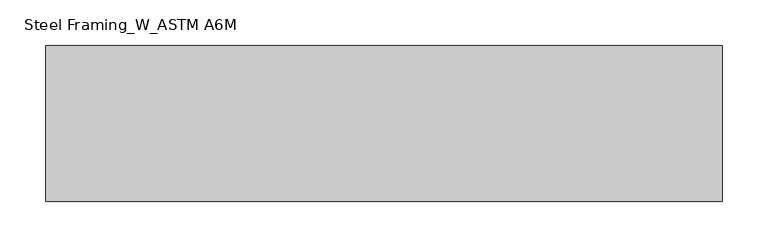
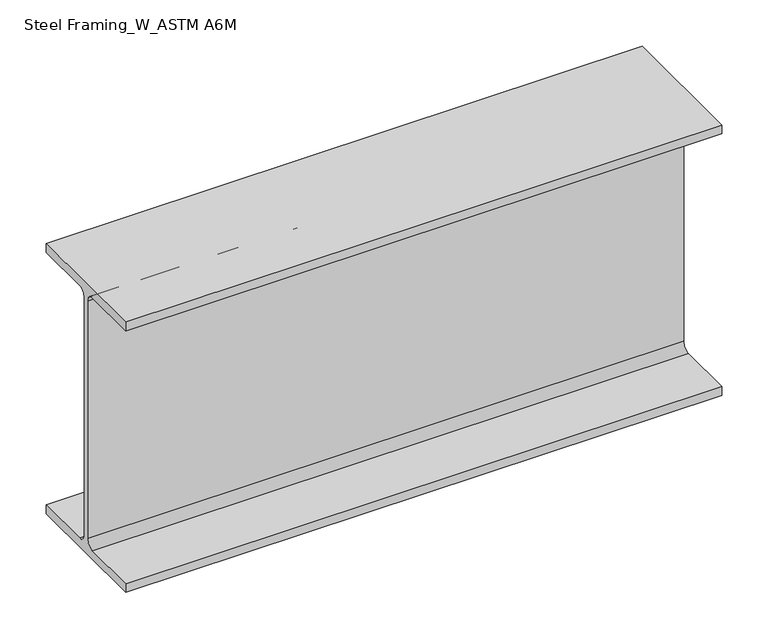
"""IFC4 building model written with IfcOpenShell, lengths in millimetres: beam geometry, Steel Framing_W_ASTM A6M : H_SB_AR_S02_W360x51_RG1."""

from ifc_helpers import new_model, si_unit, point, frame, frame_2d, origin, place, context, project, spatial, polyline, circle_curve, trimmed, segment, composite_curve, outline, extrude, source, transform, mapped, element, save


def steel_framing_w_astm_a6m_e2cb39de(model_context):
    return source(origin(), model_context, "Body", "SweptSolid", [
        extrude(outline(composite_curve([segment(polyline([(85.5, -166.4), (85.5, -178.0), (-85.5, -178.0), (-85.5, -166.4), (-13.72, -166.4)]), True, "CONTINUOUS"), segment(trimmed(circle_curve(frame_2d((-13.72, -156.3)), 10.1), [point((-13.72, -166.4))], [point((-3.62, -156.3))], True, "CARTESIAN"), True, "CONTINUOUS"), segment(polyline([(-3.62, -156.3), (-3.62, 156.3)]), True, "CONTINUOUS"), segment(trimmed(circle_curve(frame_2d((-13.72, 156.3)), 10.1), [point((-3.62, 156.3))], [point((-13.72, 166.4))], True, "CARTESIAN"), True, "CONTINUOUS"), segment(polyline([(-13.72, 166.4), (-85.5, 166.4), (-85.5, 178.0), (85.5, 178.0), (85.5, 166.4), (13.72, 166.4)]), True, "CONTINUOUS"), segment(trimmed(circle_curve(frame_2d((13.72, 156.3)), 10.1), [point((13.72, 166.4))], [point((3.62, 156.3))], True, "CARTESIAN"), True, "CONTINUOUS"), segment(polyline([(3.62, 156.3), (3.62, -156.3)]), True, "CONTINUOUS"), segment(trimmed(circle_curve(frame_2d((13.72, -156.3)), 10.1), [point((3.62, -156.3))], [point((13.72, -166.4))], True, "CARTESIAN"), True, "CONTINUOUS"), segment(polyline([(13.72, -166.4), (85.5, -166.4)]), True, "CONTINUOUS")], self_intersect=False)), frame((-229.55, 0.0, 0.0), z_axis=(1.0, 0.0, 0.0), x_axis=(0.0, 1.0, 0.0)), (0.0, 0.0, 1.0), 742.1),
    ])


if __name__ == "__main__":
    model = new_model("IFC4")
    model_context = context("Model", 3, world=origin())
    ifc_project = project(units=[si_unit("LENGTHUNIT", "METRE", prefix="MILLI")], contexts=[model_context])
    site = spatial("IfcSite", under=ifc_project)
    building = spatial("IfcBuilding", under=site)
    placement = place(None, origin())
    steel_framing_w_astm_a6m_shape = steel_framing_w_astm_a6m_e2cb39de(model_context)
    element("IfcBeam", 1, ObjectType="Steel Framing_W_ASTM A6M : H_SB_AR_S02_W360x51_RG1", at=placement, inside=building, context=model_context, shape_type="MappedRepresentation", body=[
        mapped(steel_framing_w_astm_a6m_shape, transform((0.0, 0.0, 0.0), x_axis=(1.0, 0.0, 0.0), y_axis=(0.0, 1.0, 0.0), z_axis=(0.0, 0.0, 1.0))),
    ])
    save(model, "model.ifc")

# Revit data of these elements
# Type "Steel Framing_W_ASTM A6M : H_SB_AR_S02_W360x51_RG1"
#   Type Mark = "RG1"
#   Section Name Key = "W14x34"
#   Width = 17.1 cm
#   Web Thickness = 0.724 cm
#   Web Fillet = 1.01 cm
#   Warping Constant = 287000.0 cm⁶
#   Torsional Moment of Inertia = 23.70 cm⁴
#   Section Area = 64.5 cm²
#   Plastic Modulus weak axis = 174.0 cm³
#   Plastic Modulus strong axis = 895.0 cm³
#   Perimeter = 1.36 m²/m
#   Nominal Weight = 51.00 kgf/m
#   Moment of Inertia weak axis = 970.00 cm⁴
#   Moment of Inertia strong axis = 14200.00 cm⁴
#   Height = 35.6 cm
#   Flange Thickness = 1.16 cm
#   Elastic Modulus weak axis = 113.0 cm³
#   Elastic Modulus strong axis = 796.0 cm³
#   Centroid Vertical = 17.8 cm
#   Centroid Horizontal = 8.55 cm
#   Length [instance default] = 1500 mm
#   Structural Material [instance default] = Steel, 45-345
#   Bolt Spacing = 0
#   Assembly Code = ""
# Element 1 (IfcBeam, "Steel Framing_W_ASTM A6M : H_SB_AR_S02_W360x51_RG1")
#   Materials on its faces: "Steel, 45-345"
# Materials
#   "Steel, 45-345": class "Metal", colour RGB 189 187 185, transparency 0, Description = "Steel 345 MPa", Cost = 0
